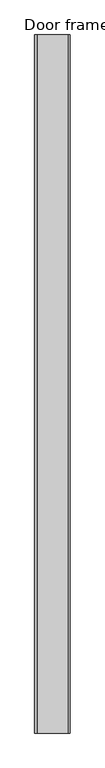
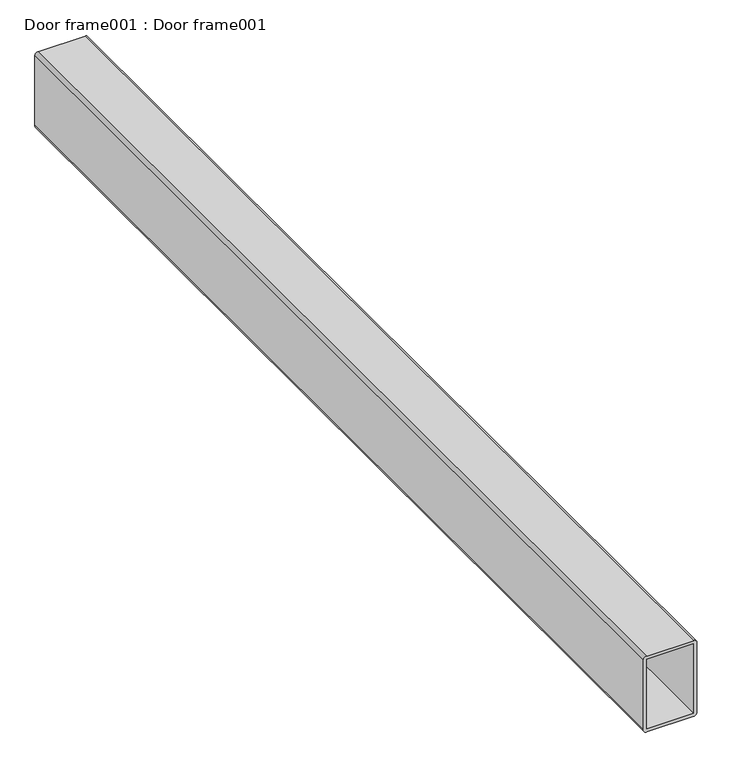
"""IFC4 building model written with IfcOpenShell, lengths in millimetres: proxy geometry, Door frame001 : Door frame001."""

from ifc_helpers import new_model, si_unit, point, frame, frame_2d, origin, place, context, project, spatial, polyline, circle_curve, trimmed, segment, composite_curve, outline, extrude, source, transform, mapped, element, save


def door_frame001_door_frame001_2a17c90b(model_context):
    return source(origin(), model_context, "Body", "SweptSolid", [
        extrude(outline(composite_curve([segment(polyline([(32616.0375625, -8390.3106967), (32616.0375625, -8301.4106967)]), True, "CONTINUOUS"), segment(trimmed(circle_curve(frame_2d((32622.3875625, -8301.4106967)), 6.35), [point((32616.0375625, -8301.4106967))], [point((32622.3875625, -8295.0606967))], False, "CARTESIAN"), True, "CONTINUOUS"), segment(polyline([(32622.3875625, -8295.0606967), (32762.0875625, -8295.0606967)]), True, "CONTINUOUS"), segment(trimmed(circle_curve(frame_2d((32762.0875625, -8301.4106967)), 6.35), [point((32762.0875625, -8295.0606967))], [point((32768.4375625, -8301.4106967))], False, "CARTESIAN"), True, "CONTINUOUS"), segment(polyline([(32768.4375625, -8301.4106967), (32768.4375625, -8390.3106967)]), True, "CONTINUOUS"), segment(trimmed(circle_curve(frame_2d((32762.0875625, -8390.3106967)), 6.35), [point((32768.4375625, -8390.3106967))], [point((32762.0875625, -8396.6606967))], False, "CARTESIAN"), True, "CONTINUOUS"), segment(polyline([(32762.0875625, -8396.6606967), (32622.3875625, -8396.6606967)]), True, "CONTINUOUS"), segment(trimmed(circle_curve(frame_2d((32622.3875625, -8390.3106967)), 6.35), [point((32622.3875625, -8396.6606967))], [point((32616.0375625, -8390.3106967))], False, "CARTESIAN"), True, "CONTINUOUS")], self_intersect=False), holes=[polyline([(32761.9375625, -8301.5606967), (32622.5375625, -8301.5606967), (32622.5375625, -8390.1606967), (32761.9375625, -8390.1606967), (32761.9375625, -8301.5606967)])]), frame((0.0, 4540.4513244, 0.0), z_axis=(0.0, 1.0, 0.0), x_axis=(0.0, 0.0, 1.0)), (0.0, 0.0, 1.0), 2000.0),
    ])


if __name__ == "__main__":
    model = new_model("IFC4")
    model_context = context("Model", 3, world=origin())
    ifc_project = project(units=[si_unit("LENGTHUNIT", "METRE", prefix="MILLI")], contexts=[model_context])
    site = spatial("IfcSite", under=ifc_project)
    building = spatial("IfcBuilding", under=site)
    placement = place(None, origin())
    door_frame001_door_frame001_shape = door_frame001_door_frame001_2a17c90b(model_context)
    element("IfcBuildingElementProxy", 1, Name="Door frame001 : Door frame001", ObjectType="Door frame001 : Door frame001", at=placement, inside=building, context=model_context, shape_type="MappedRepresentation", body=[
        mapped(door_frame001_door_frame001_shape, transform((0.0, 0.0, 0.0), x_axis=(1.0, 0.0, 0.0), y_axis=(0.0, 1.0, 0.0), z_axis=(0.0, 0.0, 1.0))),
    ])
    save(model, "model.ifc")

# Revit data of these elements
# Type "Door frame001 : Door frame001"
#   NameOverride = "Door frame001"
# Element 1 (IfcBuildingElementProxy, "Door frame001 : Door frame001")
#   Materials on its faces: "DOOR FRAME: TUBE STEEL PROFILE - METALIZED, PRIMED & PAINTED (COLOR PER ARCHITECT)"
# Materials
#   "DOOR FRAME: TUBE STEEL PROFILE - METALIZED, PRIMED & PAINTED (COLOR PER ARCHITECT)": class "Unassigned", colour RGB 128 128 128, transparency 0, Cost = 0
